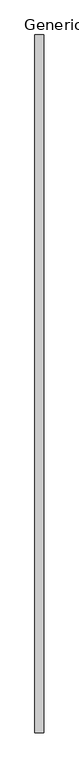
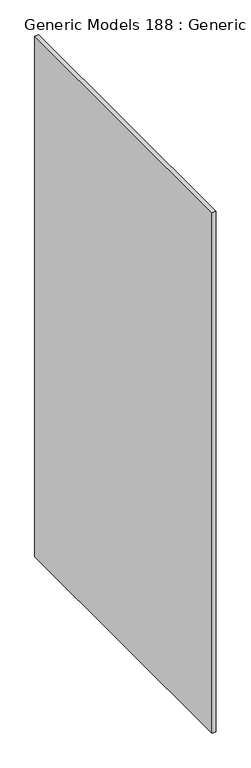
"""IFC4 building model written with IfcOpenShell, lengths in millimetres: proxy geometry, Generic Models 188 : Generic Models 1."""

from ifc_helpers import new_model, si_unit, frame, origin, place, context, project, spatial, polyline, outline, extrude, source, transform, mapped, element, save


def generic_models_188_generic_models_1_1a6d81a6(model_context):
    return source(origin(), model_context, "Body", "SweptSolid", [
        extrude(outline(polyline([(47361.475, 1219.2), (47361.475, 0.0), (47345.6, 0.0), (47345.6, 1219.2), (47361.475, 1219.2)])), frame((0.0, 0.0, 6.35), z_axis=(0.0, 0.0, 1.0), x_axis=(1.0, 0.0, 0.0)), (0.0, 0.0, 1.0), 2181.8704978),
    ])


if __name__ == "__main__":
    model = new_model("IFC4")
    model_context = context("Model", 3, world=origin())
    ifc_project = project(units=[si_unit("LENGTHUNIT", "METRE", prefix="MILLI")], contexts=[model_context])
    site = spatial("IfcSite", under=ifc_project)
    building = spatial("IfcBuilding", under=site)
    placement = place(None, origin())
    generic_models_188_generic_models_1_shape = generic_models_188_generic_models_1_1a6d81a6(model_context)
    element("IfcBuildingElementProxy", 1, Name="Generic Models 188 : Generic Models 1", ObjectType="Generic Models 188 : Generic Models 1", at=placement, inside=building, context=model_context, shape_type="MappedRepresentation", body=[
        mapped(generic_models_188_generic_models_1_shape, transform((0.0, 0.0, 0.0), x_axis=(1.0, 0.0, 0.0), y_axis=(0.0, 1.0, 0.0), z_axis=(0.0, 0.0, 1.0))),
    ])
    save(model, "model.ifc")

# Revit data of these elements
# Element 1 (IfcBuildingElementProxy, "Generic Models 188 : Generic Models 1")
#   Materials on its faces: "GYP. BD (SEE 'WALL TAG' & 'LAYER MATERIAL SCHEDULE' FOR DETAILS)"
# Materials
#   "GYP. BD (SEE 'WALL TAG' & 'LAYER MATERIAL SCHEDULE' FOR DETAILS)": class "Generic", colour RGB 237 236 233, transparency 0, Description = "Gypsum Wall Board", Cost = 0
